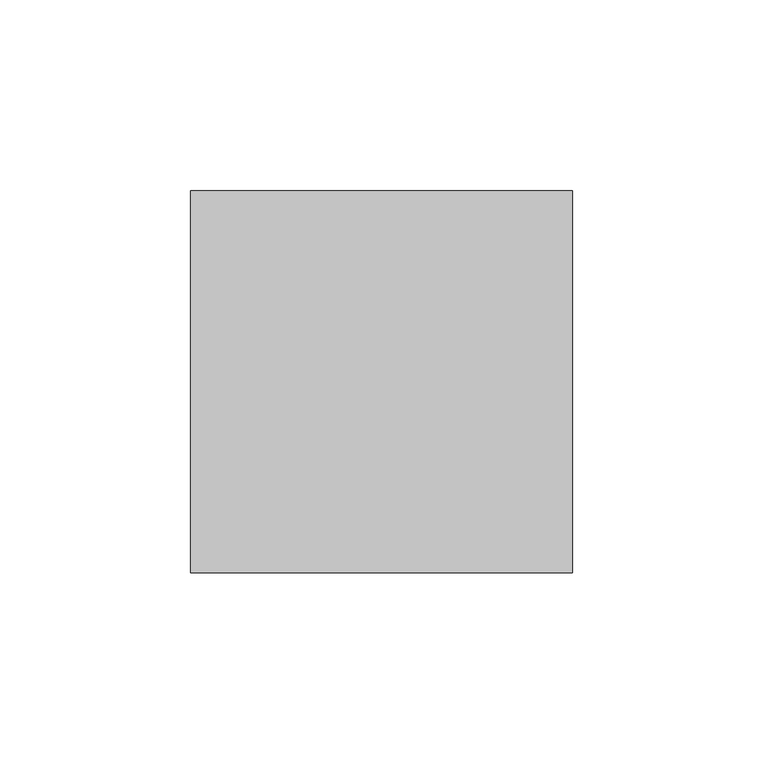
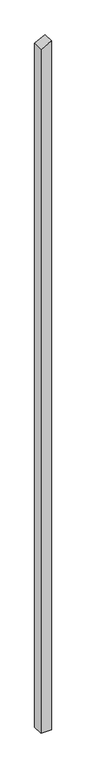
"""IFC4 building model written with IfcOpenShell, lengths in millimetres: column geometry, Holzstütze 159906 : Holzstütze 159906."""

import ifcopenshell
import ifcopenshell.guid

model = None  # the IFC model being written
_history = None  # IfcOwnerHistory: only IFC2X3 demands one
_inside = {}  # id of a spatial element -> (the spatial element, [elements in it])
_under = {}  # id of a project, library or spatial element -> (it, [spatial elements below it])
_declared = {}  # id of a project -> (the project, [libraries it declares])
_typed = {}  # id of a type object -> (the type object, [elements of that type])
_made_of = {}  # id of a material, layer set ... -> (it, [elements and type objects made of it])


def new_model(schema):
    """Start an empty IFC model of exactly this schema.

    Asked for "IFC4X3", IfcOpenShell would pick the latest addendum, in which some entities
    have other attributes; the version numbers below select the first issue.
    IFC2X3 requires an IfcOwnerHistory on every rooted entity: one is made here for all.
    """
    global model, _history
    if schema == "IFC4X3":
        model = ifcopenshell.file(schema_version=(4, 3, 0, 0))
    else:
        model = ifcopenshell.file(schema=schema)
    _inside.clear()
    _under.clear()
    _declared.clear()
    _typed.clear()
    _made_of.clear()
    _history = None
    if model.schema == "IFC2X3":
        org = make("IfcOrganization", Name="unknown")
        user = make(
            "IfcPersonAndOrganization",
            ThePerson=make("IfcPerson", FamilyName="unknown"),
            TheOrganization=org,
        )
        app = make(
            "IfcApplication",
            ApplicationDeveloper=org,
            Version="unknown",
            ApplicationFullName="unknown",
            ApplicationIdentifier="unknown",
        )
        _history = make(
            "IfcOwnerHistory",
            OwningUser=user,
            OwningApplication=app,
            ChangeAction="ADDED",
            CreationDate=0,
        )
    return model


def make(cls, **values):
    """One entity of the class cls with the attributes given. An attribute that is None is left unset."""
    return model.create_entity(
        cls, **{name: value for name, value in values.items() if value is not None}
    )


def rooted(cls, **values):
    """An entity with a GlobalId (a new one), such as an element, a storey or a relation."""
    return make(cls, GlobalId=ifcopenshell.guid.new(), OwnerHistory=_history, **values)


def si_unit(unit_type, name, prefix=None):
    """IfcSIUnit, for example si_unit("LENGTHUNIT", "METRE", prefix="MILLI")."""
    return make("IfcSIUnit", UnitType=unit_type, Prefix=prefix, Name=name)


def assignment(units):
    """IfcUnitAssignment: the units of a project."""
    return None if units is None else make("IfcUnitAssignment", Units=units)


def point(xyz):
    """IfcCartesianPoint."""
    return None if xyz is None else make("IfcCartesianPoint", Coordinates=xyz)


def direction(xyz):
    """IfcDirection."""
    return None if xyz is None else make("IfcDirection", DirectionRatios=xyz)


def frame(location, z_axis=None, x_axis=None):
    """IfcAxis2Placement3D, a coordinate frame: its origin and axes. An axis left out is left unset."""
    return make(
        "IfcAxis2Placement3D",
        Location=point(location),
        Axis=direction(z_axis),
        RefDirection=direction(x_axis),
    )


def origin():
    """The frame at (0, 0, 0) with its axes left unset."""
    return frame((0.0, 0.0, 0.0))


def place(relative_to, where):
    """IfcLocalPlacement: puts the frame where relative to a parent placement (None: the world)."""
    return make(
        "IfcLocalPlacement", PlacementRelTo=relative_to, RelativePlacement=where
    )


def context(
    kind, dimensions, precision=None, world=None, true_north=None, identifier=None
):
    """IfcGeometricRepresentationContext, for example the 3D "Model" context."""
    return make(
        "IfcGeometricRepresentationContext",
        ContextIdentifier=identifier,
        ContextType=kind,
        CoordinateSpaceDimension=dimensions,
        Precision=precision,
        WorldCoordinateSystem=world,
        TrueNorth=true_north,
    )


def project(units=None, contexts=None):
    """IfcProject with its units and contexts."""
    return rooted(
        "IfcProject",
        Name="project",
        RepresentationContexts=contexts,
        UnitsInContext=assignment(units),
    )


def spatial(cls, under=None, at=None, **own):
    """A site, building, storey or space (cls), placed at a placement, below another one or the project."""
    s = rooted(cls, ObjectPlacement=at, **own)
    if under is not None:
        _under.setdefault(under.id(), (under, []))[1].append(s)
    return s


def polyline(points):
    """IfcPolyline through the points."""
    return make("IfcPolyline", Points=[point(p) for p in points])


def outline(outer, holes=None, kind="AREA"):
    """IfcArbitraryClosedProfileDef: a profile drawn as a closed curve; with holes, ...WithVoids."""
    if holes is None:
        return make("IfcArbitraryClosedProfileDef", ProfileType=kind, OuterCurve=outer)
    return make(
        "IfcArbitraryProfileDefWithVoids",
        ProfileType=kind,
        OuterCurve=outer,
        InnerCurves=holes,
    )


def extrude(swept, where, along, depth):
    """IfcExtrudedAreaSolid: the profile swept, set in the frame where, extruded along a direction by depth."""
    return make(
        "IfcExtrudedAreaSolid",
        SweptArea=swept,
        Position=where,
        ExtrudedDirection=direction(along),
        Depth=depth,
    )


def shape(context_of_items, identifier, shape_type, items):
    """IfcShapeRepresentation: the items that make up one representation, for example the "Body"."""
    return make(
        "IfcShapeRepresentation",
        ContextOfItems=context_of_items,
        RepresentationIdentifier=identifier,
        RepresentationType=shape_type,
        Items=items,
    )


def source(mapping_origin, context_of_items, identifier, shape_type, items):
    """IfcRepresentationMap: a shape defined once, which mapped items show again and again."""
    return make(
        "IfcRepresentationMap",
        MappingOrigin=mapping_origin,
        MappedRepresentation=shape(context_of_items, identifier, shape_type, items),
    )


def transform(
    local_origin,
    x_axis=None,
    y_axis=None,
    z_axis=None,
    scale=None,
    scale2=None,
    scale3=None,
    uniform=True,
):
    """IfcCartesianTransformationOperator3D, or its non-uniform kind. x_axis, y_axis, z_axis: its Axis1, 2, 3."""
    if uniform:
        return make(
            "IfcCartesianTransformationOperator3D",
            Axis1=direction(x_axis),
            Axis2=direction(y_axis),
            LocalOrigin=point(local_origin),
            Scale=scale,
            Axis3=direction(z_axis),
        )
    return make(
        "IfcCartesianTransformationOperator3DnonUniform",
        Axis1=direction(x_axis),
        Axis2=direction(y_axis),
        LocalOrigin=point(local_origin),
        Scale=scale,
        Axis3=direction(z_axis),
        Scale2=scale2,
        Scale3=scale3,
    )


def mapped(mapping_source, mapping_target):
    """IfcMappedItem: shows the shape of a source again, moved by a transform."""
    return make(
        "IfcMappedItem", MappingSource=mapping_source, MappingTarget=mapping_target
    )


def made_of(thing, what):
    """Note that an element or type object is made of a material, layer set ...; save() writes the relation."""
    if what is not None:
        _made_of.setdefault(what.id(), (what, []))[1].append(thing)
    return thing


def element(
    cls,
    number,
    at=None,
    inside=None,
    cuts=None,
    type_object=None,
    material=None,
    context=None,
    identifier="Body",
    shape_type=None,
    held_by="IfcProductDefinitionShape",
    body=None,
    shapes=None,
    **own,
):
    """One element of the class cls, such as IfcWall. Its Tag is "e" and its number.

    at: its placement. inside: the storey or other place that contains it. cuts: it is an
    opening in that element (IfcRelVoidsElement). A single representation is given by context,
    identifier, shape_type and body (its items); several are given by shapes. held_by: the class
    of the entity that holds the representations. save() writes the other relations.
    """
    e = rooted(cls, Tag="e%d" % number, ObjectPlacement=at, **own)
    if body is not None:
        shapes = [shape(context, identifier, shape_type, body)]
    if shapes is not None:
        e.Representation = make(held_by, Representations=shapes)
    if inside is not None:
        _inside.setdefault(inside.id(), (inside, []))[1].append(e)
    if cuts is not None:
        rooted(
            "IfcRelVoidsElement", RelatingBuildingElement=cuts, RelatedOpeningElement=e
        )
    if type_object is not None:
        _typed.setdefault(type_object.id(), (type_object, []))[1].append(e)
    return made_of(e, material)


def aggregate(whole, parts):
    """IfcRelAggregates: a whole, such as a stair, and the parts it consists of."""
    return rooted("IfcRelAggregates", RelatingObject=whole, RelatedObjects=parts)


def save(model, path):
    """Write the relations noted so far, then the file.

    IfcRelAggregates (storeys below a building ...), IfcRelContainedInSpatialStructure (elements
    in a storey), IfcRelDefinesByType, IfcRelAssociatesMaterial and IfcRelDeclares: one each for
    every whole, place, type object, material and project.
    """
    for whole, parts in _under.values():
        aggregate(whole, parts)
    for where, things in _inside.values():
        rooted(
            "IfcRelContainedInSpatialStructure",
            RelatedElements=things,
            RelatingStructure=where,
        )
    for kind, things in _typed.values():
        rooted("IfcRelDefinesByType", RelatedObjects=things, RelatingType=kind)
    for what, things in _made_of.values():
        rooted("IfcRelAssociatesMaterial", RelatedObjects=things, RelatingMaterial=what)
    for by, libraries in _declared.values():
        rooted("IfcRelDeclares", RelatingContext=by, RelatedDefinitions=libraries)
    model.write(path)


def column_86400a18(model_context):
    return source(origin(), model_context, "Body", "SweptSolid", [
        extrude(outline(polyline([(-500.0, 157297.7593015), (-500.0, 157397.7593015), (6396.6643707, 157397.7593015), (6345.7118258, 157297.7593015), (-500.0, 157297.7593015)])), frame((0.0, 36959.3988814, 0.0), z_axis=(0.0, 1.0, 0.0), x_axis=(0.0, 0.0, 1.0)), (0.0, 0.0, 1.0), 100.0),
    ])


if __name__ == "__main__":
    model = new_model("IFC4")
    model_context = context("Model", 3, world=origin())
    ifc_project = project(units=[si_unit("LENGTHUNIT", "METRE", prefix="MILLI")], contexts=[model_context])
    site = spatial("IfcSite", under=ifc_project)
    building = spatial("IfcBuilding", under=site)
    placement = place(None, origin())
    column_shape = column_86400a18(model_context)
    element("IfcColumn", 1, ObjectType="Holzstütze 159906 : Holzstütze 159906", at=placement, inside=building, context=model_context, shape_type="MappedRepresentation", body=[
        mapped(column_shape, transform((0.0, 0.0, 0.0), x_axis=(1.0, 0.0, 0.0), y_axis=(0.0, 1.0, 0.0), z_axis=(0.0, 0.0, 1.0))),
    ])
    save(model, "model.ifc")

# Revit data of these elements
# Type "Holzstütze 159906 : Holzstütze 159906"
#   Abrechnungsart = "m"
#   Allright_Bauteil_ID = "0152St 0000143509"
#   Bezeichnung = "Holzstütze"
#   Codetext = "ST-HOLZ\\"
#   Gewerk = "Zimmer- und Holzbauarbeiten"
#   Material = "Holz"
#   Objektname = "Stütze"
#   NameOverride = "Holzstütze"
#   Reference = "Holzstütze"
#   Status = "NEW"
#   ThermalTransmittance = 0.0000 BTU/(h·ft²·°F)
#   Roll = 0.00°
#   Slope = 0.00°
#   2D Interaktion = yes
#   IsExternal = yes
#   LoadBearing = yes
# Element 1 (IfcColumn, "Holzstütze 159906 : Holzstütze 159906")
#   Materials on its faces: "holzschalung"
# Materials
#   "holzschalung": class "Unassigned", colour RGB 128 128 128, transparency 0
